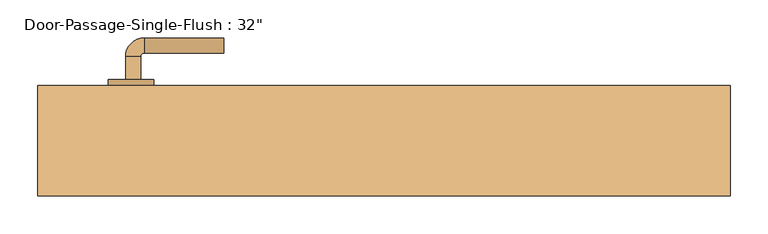
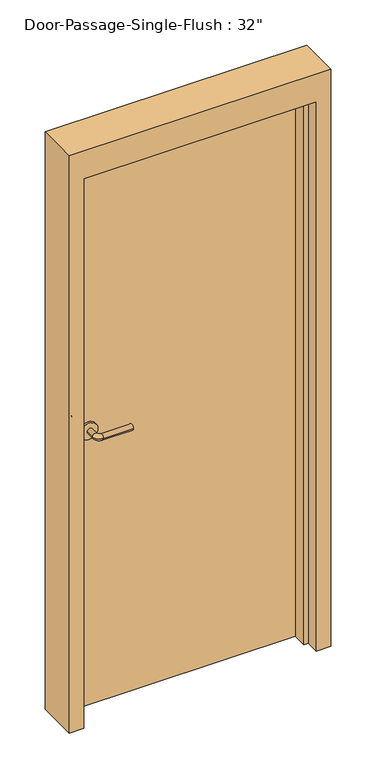
"""IFC4 building model written with IfcOpenShell, lengths in millimetres: door geometry."""

from ifc_helpers import new_model, si_unit, point, frame, frame_2d, origin, origin_with_axes, place, context, project, spatial, polyline, circle_curve, ellipse_curve, trimmed, segment, composite_curve, outline, extrude, faceted_brep, source, transform, mapped, element, save
from ifc_brep_helpers import plane_surface, cylinder_surface, revolved_surface, advanced_brep


def door_c58a95c4(model_context):
    return source(origin(), model_context, "Body", "SolidModel", [
        advanced_brep(
        [(-341.390625, -11.175, 1016.0), (-321.390625, -11.175, 1016.0), (-321.390625, -41.175, 1016.0), (-341.390625, -41.175, 1016.0), (-316.390625, -46.175, 1016.0), (-316.390625, -66.175, 1016.0), (-211.390625, -66.175, 1016.0), (-211.390625, -46.175, 1016.0)],
        [
            (0, 1, circle_curve(frame((-331.390625, -11.175, 1016.0), z_axis=(0.0, 1.0, 0.0), x_axis=(1.0, 0.0, 0.0)), 10.0)),
            (1, 0, circle_curve(frame((-331.390625, -11.175, 1016.0), z_axis=(0.0, 1.0, 0.0), x_axis=(1.0, 0.0, 0.0)), 10.0)),
            (1, 2),
            (2, 3, circle_curve(frame((-331.390625, -41.175, 1016.0), z_axis=(0.0, 1.0, 0.0), x_axis=(1.0, 0.0, 0.0)), 10.0)),
            (3, 0),
            (3, 2, circle_curve(frame((-331.390625, -41.175, 1016.0), z_axis=(0.0, 1.0, 0.0), x_axis=(1.0, 0.0, 0.0)), 10.0)),
            (4, 5, circle_curve(frame((-316.390625, -56.175, 1016.0), z_axis=(-1.0, 0.0, 0.0), x_axis=(0.0, 1.0, 0.0)), 10.0)),
            (5, 3, circle_curve(frame((-316.390625, -41.175, 1016.0), z_axis=(0.0, 0.0, -1.0), x_axis=(-1.0, 0.0, 0.0)), 25.0)),
            (2, 4, circle_curve(frame((-316.390625, -41.175, 1016.0), z_axis=(0.0, 0.0, 1.0), x_axis=(-1.0, 0.0, 0.0)), 5.0)),
            (5, 4, circle_curve(frame((-316.390625, -56.175, 1016.0), z_axis=(-1.0, 0.0, 0.0), x_axis=(0.0, 1.0, 0.0)), 10.0)),
            (6, 7, circle_curve(frame((-211.390625, -56.175, 1016.0), z_axis=(1.0, 0.0, 0.0), x_axis=(0.0, 1.0, 0.0)), 10.0)),
            (7, 6, circle_curve(frame((-211.390625, -56.175, 1016.0), z_axis=(1.0, 0.0, 0.0), x_axis=(0.0, 1.0, 0.0)), 10.0)),
            (4, 7),
            (6, 5),
        ],
        [
            plane_surface(frame((-331.390625, -11.175, 1016.0), z_axis=(0.0, 1.0, 0.0), x_axis=(0.0, 0.0, 1.0))),
            cylinder_surface(frame((-331.390625, -11.175, 1016.0), z_axis=(0.0, 1.0, 0.0), x_axis=(1.0, 0.0, 0.0)), 10.0),
            revolved_surface(trimmed(ellipse_curve(frame((-331.390625, -41.175, 1016.0), z_axis=(0.0, -1.0, 0.0), x_axis=(1.0, 0.0, 0.0)), 10.0, 10.0), [point((-341.390625, -41.175, 1016.0))], [point((-321.390625, -41.175, 1016.0))], True, "CARTESIAN"), (-316.390625, -41.175, 1016.0), (0.0, 0.0, -1.0)),
            revolved_surface(trimmed(ellipse_curve(frame((-331.390625, -41.175, 1016.0), z_axis=(0.0, -1.0, 0.0), x_axis=(1.0, 0.0, 0.0)), 10.0, 10.0), [point((-321.390625, -41.175, 1016.0))], [point((-341.390625, -41.175, 1016.0))], True, "CARTESIAN"), (-316.390625, -41.175, 1016.0), (0.0, 0.0, -1.0)),
            plane_surface(frame((-211.390625, -56.175, 1016.0), z_axis=(1.0, 0.0, 0.0), x_axis=(0.0, 0.0, 1.0))),
            cylinder_surface(frame((-316.390625, -56.175, 1016.0), z_axis=(-1.0, 0.0, 0.0), x_axis=(0.0, 1.0, 0.0)), 10.0),
        ],
        [
            (0, [[1, 2]]),
            (1, [[3, 4, 5, -2]]),
            (1, [[-5, 6, -3, -1]]),
            (2, [[7, 8, -4, 9]]),
            (3, [[10, -9, -6, -8]]),
            (4, [[11, 12]]),
            (5, [[13, -11, 14, -7]]),
            (5, [[-14, -12, -13, -10]]),
        ],
    ),
        extrude(outline(composite_curve([segment(trimmed(circle_curve(frame_2d((1016.0, -333.890625)), 30.0), [point((1016.0, -363.890625))], [point((1016.0, -303.890625))], False, "CARTESIAN"), True, "CONTINUOUS"), segment(trimmed(circle_curve(frame_2d((1016.0, -333.890625)), 30.0), [point((1016.0, -303.890625))], [point((1016.0, -363.890625))], False, "CARTESIAN"), True, "CONTINUOUS")], self_intersect=False)), frame((0.0, -11.175, 0.0), z_axis=(0.0, 1.0, 0.0), x_axis=(0.0, 0.0, 1.0)), (0.0, 0.0, 1.0), 8.0),
        advanced_brep(
        [(-341.390625, 49.275, 1016.0), (-321.390625, 49.275, 1016.0), (-341.390625, 79.275, 1016.0), (-321.390625, 79.275, 1016.0), (-316.390625, 84.275, 1016.0), (-316.390625, 104.275, 1016.0), (-211.390625, 104.275, 1016.0), (-211.390625, 84.275, 1016.0)],
        [
            (0, 1, circle_curve(frame((-331.390625, 49.275, 1016.0), z_axis=(0.0, -1.0, 0.0), x_axis=(1.0, 0.0, 0.0)), 10.0)),
            (1, 0, circle_curve(frame((-331.390625, 49.275, 1016.0), z_axis=(0.0, -1.0, 0.0), x_axis=(1.0, 0.0, 0.0)), 10.0)),
            (0, 2),
            (2, 3, circle_curve(frame((-331.390625, 79.275, 1016.0), z_axis=(0.0, -1.0, 0.0), x_axis=(1.0, 0.0, 0.0)), 10.0)),
            (3, 1),
            (3, 2, circle_curve(frame((-331.390625, 79.275, 1016.0), z_axis=(0.0, -1.0, 0.0), x_axis=(1.0, 0.0, 0.0)), 10.0)),
            (4, 3, circle_curve(frame((-316.390625, 79.275, 1016.0), z_axis=(0.0, 0.0, 1.0), x_axis=(-1.0, 0.0, 0.0)), 5.0)),
            (2, 5, circle_curve(frame((-316.390625, 79.275, 1016.0), z_axis=(0.0, 0.0, -1.0), x_axis=(-1.0, 0.0, 0.0)), 25.0)),
            (5, 4, circle_curve(frame((-316.390625, 94.275, 1016.0), z_axis=(-1.0, 0.0, 0.0), x_axis=(0.0, -1.0, 0.0)), 10.0)),
            (4, 5, circle_curve(frame((-316.390625, 94.275, 1016.0), z_axis=(-1.0, 0.0, 0.0), x_axis=(0.0, -1.0, 0.0)), 10.0)),
            (6, 7, circle_curve(frame((-211.390625, 94.275, 1016.0), z_axis=(1.0, 0.0, 0.0), x_axis=(0.0, -1.0, 0.0)), 10.0)),
            (7, 6, circle_curve(frame((-211.390625, 94.275, 1016.0), z_axis=(1.0, 0.0, 0.0), x_axis=(0.0, -1.0, 0.0)), 10.0)),
            (5, 6),
            (7, 4),
        ],
        [
            plane_surface(frame((-331.390625, 49.275, 1016.0), z_axis=(0.0, -1.0, 0.0), x_axis=(0.0, 0.0, 1.0))),
            cylinder_surface(frame((-331.390625, 49.275, 1016.0), z_axis=(0.0, -1.0, 0.0), x_axis=(1.0, 0.0, 0.0)), 10.0),
            revolved_surface(trimmed(ellipse_curve(frame((-331.390625, 79.275, 1016.0), z_axis=(0.0, -1.0, 0.0), x_axis=(1.0, 0.0, 0.0)), 10.0, 10.0), [point((-341.390625, 79.275, 1016.0))], [point((-321.390625, 79.275, 1016.0))], True, "CARTESIAN"), (-316.390625, 79.275, 1016.0), (0.0, 0.0, -1.0)),
            revolved_surface(trimmed(ellipse_curve(frame((-331.390625, 79.275, 1016.0), z_axis=(0.0, -1.0, 0.0), x_axis=(1.0, 0.0, 0.0)), 10.0, 10.0), [point((-321.390625, 79.275, 1016.0))], [point((-341.390625, 79.275, 1016.0))], True, "CARTESIAN"), (-316.390625, 79.275, 1016.0), (0.0, 0.0, -1.0)),
            plane_surface(frame((-211.390625, 94.275, 1016.0), z_axis=(1.0, 0.0, 0.0), x_axis=(0.0, 0.0, 1.0))),
            cylinder_surface(frame((-316.390625, 94.275, 1016.0), z_axis=(-1.0, 0.0, 0.0), x_axis=(0.0, -1.0, 0.0)), 10.0),
        ],
        [
            (0, [[1, 2]]),
            (1, [[-1, 3, 4, 5]]),
            (1, [[-2, -5, 6, -3]]),
            (2, [[7, -4, 8, 9]]),
            (3, [[-8, -6, -7, 10]]),
            (4, [[11, 12]]),
            (5, [[-9, 13, -12, 14]]),
            (5, [[-10, -14, -11, -13]]),
        ],
    ),
        extrude(outline(composite_curve([segment(trimmed(circle_curve(frame_2d((1016.0, -333.890625)), 30.0), [point((1016.0, -363.890625))], [point((1016.0, -303.890625))], False, "CARTESIAN"), True, "CONTINUOUS"), segment(trimmed(circle_curve(frame_2d((1016.0, -333.890625)), 30.0), [point((1016.0, -303.890625))], [point((1016.0, -363.890625))], False, "CARTESIAN"), True, "CONTINUOUS")], self_intersect=False)), frame((0.0, 41.275, 0.0), z_axis=(0.0, 1.0, 0.0), x_axis=(0.0, 0.0, 1.0)), (0.0, 0.0, 1.0), 8.0),
        faceted_brep([(406.4, -7.9375, 0.0), (406.4, 41.275, 0.0), (457.2, 41.275, 0.0), (457.2, -104.775, 0.0), (406.4, -104.775, 0.0), (406.4, -55.5625, 0.0), (390.525, -55.5625, 0.0), (390.525, -7.9375, 0.0), (406.4, -7.9375, 2032.0), (406.4, 41.275, 2032.0), (-406.4, 41.275, 2032.0), (-406.4, 41.275, 0.0), (-457.2, 41.275, 0.0), (-457.2, 41.275, 2133.6), (457.2, 41.275, 2133.6), (457.2, -104.775, 2133.6), (-457.2, -104.775, 2133.6), (-457.2, -104.775, 0.0), (-406.4, -104.775, 0.0), (-406.4, -104.775, 2032.0), (406.4, -104.775, 2032.0), (406.4, -55.5625, 2032.0), (-406.4, -55.5625, 2032.0), (-406.4, -55.5625, 0.0), (-390.525, -55.5625, 0.0), (-390.525, -55.5625, 2016.125), (390.525, -55.5625, 2016.125), (390.525, -7.9375, 2016.125), (-390.525, -7.9375, 2016.125), (-390.525, -7.9375, 0.0), (-406.4, -7.9375, 0.0), (-406.4, -7.9375, 2032.0)], [[[0, 1, 2, 3, 4, 5, 6, 7]], [[1, 0, 8, 9]], [[2, 1, 9, 10, 11, 12, 13, 14]], [[3, 2, 14, 15]], [[4, 3, 15, 16, 17, 18, 19, 20]], [[5, 4, 20, 21]], [[6, 5, 21, 22, 23, 24, 25, 26]], [[7, 6, 26, 27]], [[0, 7, 27, 28, 29, 30, 31, 8]], [[9, 8, 31, 10]], [[20, 19, 22, 21]], [[26, 25, 28, 27]], [[12, 11, 30, 29, 24, 23, 18, 17]], [[11, 10, 31, 30]], [[13, 12, 17, 16]], [[19, 18, 23, 22]], [[25, 24, 29, 28]], [[15, 14, 13, 16]]]),
        extrude(outline(polyline([(406.4, -3.175), (-406.4, -3.175), (-406.4, 41.275), (406.4, 41.275), (406.4, -3.175)])), origin_with_axes(), (0.0, 0.0, 1.0), 2032.0),
    ])


if __name__ == "__main__":
    model = new_model("IFC4")
    model_context = context("Model", 3, world=origin())
    ifc_project = project(units=[si_unit("LENGTHUNIT", "METRE", prefix="MILLI")], contexts=[model_context])
    site = spatial("IfcSite", under=ifc_project)
    building = spatial("IfcBuilding", under=site)
    placement = place(None, origin())
    door_shape = door_c58a95c4(model_context)
    element("IfcDoor", 1, ObjectType="Door-Passage-Single-Flush : 32\"", at=placement, inside=building, context=model_context, shape_type="MappedRepresentation", body=[
        mapped(door_shape, transform((0.0, 0.0, 0.0), x_axis=(1.0, 0.0, 0.0), y_axis=(0.0, 1.0, 0.0), z_axis=(0.0, 0.0, 1.0))),
    ])
    save(model, "model.ifc")

# Revit data of these elements
# Type "Door-Passage-Single-Flush : 32\""
#   Type Mark = "D10"
#   Assembly Code = "B2030200"
#   Analytic Construction = "Wooden"
#   Thickness = 0' - 1 3/4"
#   Thermal Resistance (R) = 0.455703 (m²·K)/W
#   Swing Angle [instance default] = 90.00°
#   Strike Height = 3' - 4"
#   Rough Width [instance default] = 3' - 0"
#   Rough Height [instance default] = 7' - 0"
#   MF Opening Height [instance default] = 0' - 4"
#   MF Opening Width [instance default] = 0' - 4"
#   Inset Calculate [instance default] = 0' - 4"
#   Masonry Inset [instance default] = 0' - 1"
#   Height = 6' - 8"
#   Width = 2' - 8"
#   Heat Transfer Coefficient (U) = 2.19465 W/(m²·K)
#   Masonry Frame Depth = 0' - 5 3/4"
#   Masonry Frame [instance default] = yes
#   Function = 1
#   Dry Wall Frame [instance default] = no
#   Panel Material = Wood - Birch
#   Frame Material = Metal - Paint Finish - Grey
#   Door Handle Material = Aluminum
#   Visual Light Transmittance = 0
#   Solar Heat Gain Coefficient = 0
#   Wall Closure = (empty or 0)
# Element 1 (IfcDoor, "Door-Passage-Single-Flush : 32\"")
#   Materials on its faces: "Aluminum", "Metal - Paint Finish - Grey", "Wood - Birch"
# Materials
#   "Wood - Birch": class "Wood", colour RGB 166 116 52, transparency 0, Cost = 0
#   "Metal - Paint Finish - Grey": class "Paint", colour RGB 104 104 104, transparency 0, Cost = 0
#   "Aluminum": class "Metal", colour RGB 247 247 247, transparency 0, Description = "Aluminum 6061", Cost = 0
